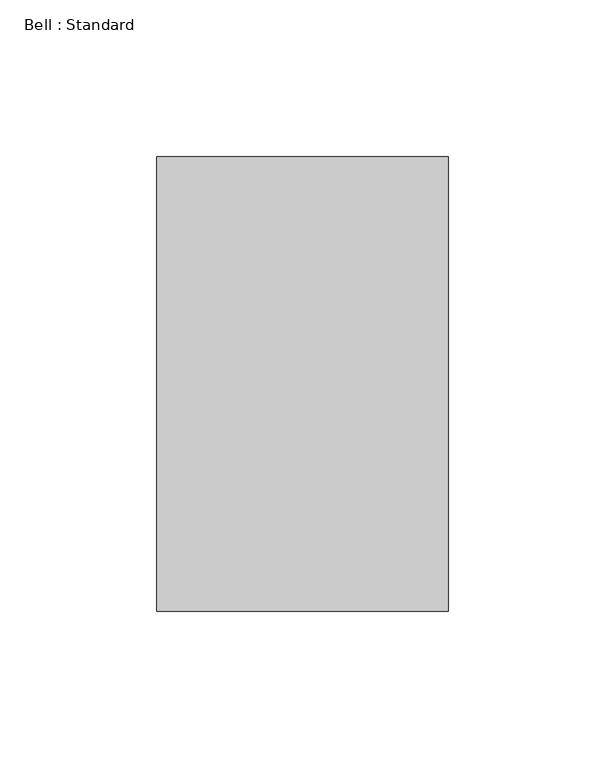
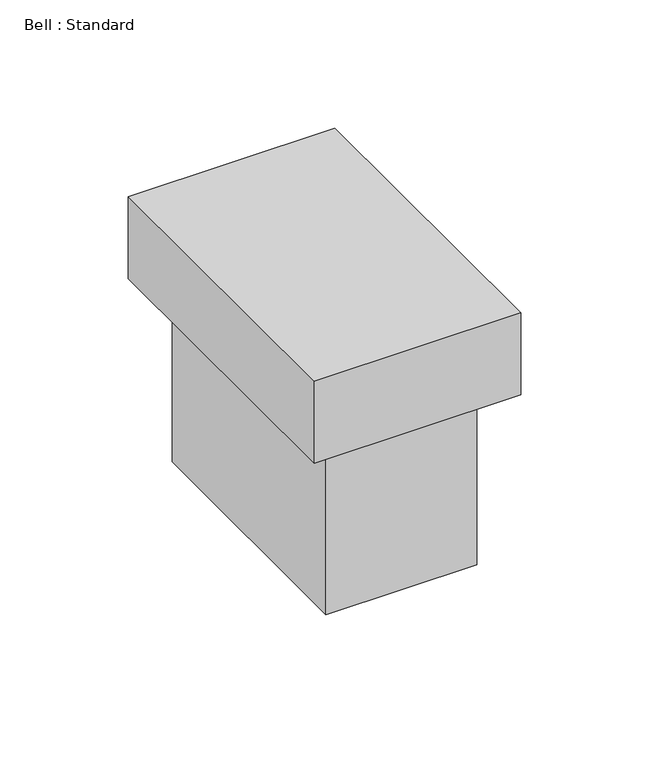
"""IFC4 building model written with IfcOpenShell, lengths in millimetres: proxy geometry, Bell : Standard."""

from ifc_helpers import new_model, si_unit, frame, origin, origin_with_axes, place, context, project, spatial, polyline, outline, extrude, source, transform, mapped, element, save


def bell_standard_b2399fa3(model_context):
    return source(origin(), model_context, "Body", "SweptSolid", [
        extrude(outline(polyline([(46.5, -145.0), (-46.5, -145.0), (-46.5, 0.0), (46.5, 0.0), (46.5, -145.0)])), origin_with_axes(), (0.0, 0.0, 1.0), 39.0),
        extrude(outline(polyline([(34.0, -132.5), (-34.0, -132.5), (-34.0, -12.5), (34.0, -12.5), (34.0, -132.5)])), frame((0.0, 0.0, -84.0286528), z_axis=(0.0, 0.0, 1.0), x_axis=(1.0, 0.0, 0.0)), (0.0, 0.0, 1.0), 84.0286528),
    ])


if __name__ == "__main__":
    model = new_model("IFC4")
    model_context = context("Model", 3, world=origin())
    ifc_project = project(units=[si_unit("LENGTHUNIT", "METRE", prefix="MILLI")], contexts=[model_context])
    site = spatial("IfcSite", under=ifc_project)
    building = spatial("IfcBuilding", under=site)
    placement = place(None, origin())
    bell_standard_shape = bell_standard_b2399fa3(model_context)
    element("IfcBuildingElementProxy", 1, Name="Bell : Standard", ObjectType="Bell : Standard", at=placement, inside=building, context=model_context, shape_type="MappedRepresentation", body=[
        mapped(bell_standard_shape, transform((0.0, 0.0, 0.0), x_axis=(1.0, 0.0, 0.0), y_axis=(0.0, 1.0, 0.0), z_axis=(0.0, 0.0, 1.0))),
    ])
    save(model, "model.ifc")

# Revit data of these elements
# Type "Bell : Standard"
#   Type Mark = "Bell"
#   Classification.OmniClass.21.Number = "21-04 70"
#   Classification.MasterFormat.Description = "Electronic Access Control and Intrusion Detection"
#   Classification.OmniClass.21.Description = "Electronic Safety and Security"
#   Classification.UniFormat.II.Description = "Access Control and Intrusion Detection"
#   Classification.MasterFormat.Number = "28 10 00"
#   Classification.OmniClass.23.Number = "23-29 11 25 19"
#   Classification.OmniClass.23.Description = "Security Buzzers"
#   Classification.UniFormat.II.Number = "D7010"
#   COBie.Type.CreatedBy = "info@mma.ie"
#   COBie.Type.CreatedOn = "2017-07-26T09:12:44"
#   COBie.Type.Name = "Bell"
#   COBie.Type.Category = "23-29 11 25 19 : Security Buzzers"
#   COBie.Type.Description = "Bell_Standard"
#   COBie.Type.AssetType = "Fixed"
#   COBie.Type.Manufacturer = ""
#   COBie.Type.ModelNumber = ""
#   COBie.Type.WarrantyDescription = ""
#   COBie.Type.ModelReference = ""
#   COBie.Type.Color = "Silver"
#   Units = "Volts"
#   Keynote = "28 13 00.A"
#   Assembly Code = "D5030400"
#   COBie.Type.ReplacementCost = 0
#   Default Elevation = 1200 mm
#   Bell_Width = 93 mm
#   Bell_Height = 145 mm
#   Bell_Depth = 39 mm
#   COBie.Type = yes
#   URL = ""
#   Type Comments = ""
#   Model = ""
#   Manufacturer = ""
